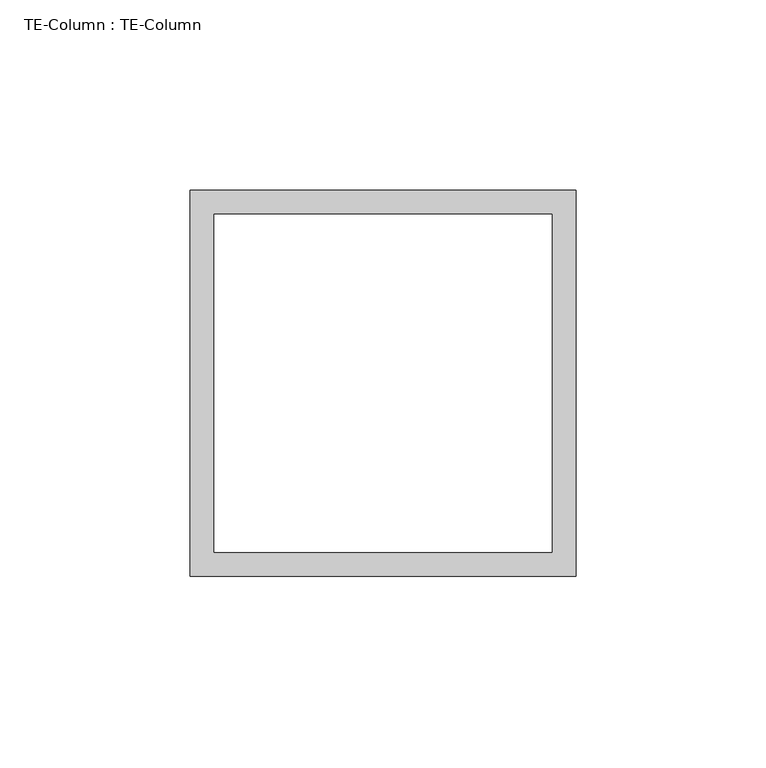
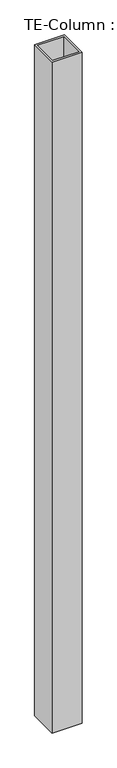
"""IFC4 building model written with IfcOpenShell, lengths in millimetres: proxy geometry, TE-Column : TE-Column."""

import ifcopenshell
import ifcopenshell.guid

model = None  # the IFC model being written
_history = None  # IfcOwnerHistory: only IFC2X3 demands one
_inside = {}  # id of a spatial element -> (the spatial element, [elements in it])
_under = {}  # id of a project, library or spatial element -> (it, [spatial elements below it])
_declared = {}  # id of a project -> (the project, [libraries it declares])
_typed = {}  # id of a type object -> (the type object, [elements of that type])
_made_of = {}  # id of a material, layer set ... -> (it, [elements and type objects made of it])


def new_model(schema):
    """Start an empty IFC model of exactly this schema.

    Asked for "IFC4X3", IfcOpenShell would pick the latest addendum, in which some entities
    have other attributes; the version numbers below select the first issue.
    IFC2X3 requires an IfcOwnerHistory on every rooted entity: one is made here for all.
    """
    global model, _history
    if schema == "IFC4X3":
        model = ifcopenshell.file(schema_version=(4, 3, 0, 0))
    else:
        model = ifcopenshell.file(schema=schema)
    _inside.clear()
    _under.clear()
    _declared.clear()
    _typed.clear()
    _made_of.clear()
    _history = None
    if model.schema == "IFC2X3":
        org = make("IfcOrganization", Name="unknown")
        user = make(
            "IfcPersonAndOrganization",
            ThePerson=make("IfcPerson", FamilyName="unknown"),
            TheOrganization=org,
        )
        app = make(
            "IfcApplication",
            ApplicationDeveloper=org,
            Version="unknown",
            ApplicationFullName="unknown",
            ApplicationIdentifier="unknown",
        )
        _history = make(
            "IfcOwnerHistory",
            OwningUser=user,
            OwningApplication=app,
            ChangeAction="ADDED",
            CreationDate=0,
        )
    return model


def make(cls, **values):
    """One entity of the class cls with the attributes given. An attribute that is None is left unset."""
    return model.create_entity(
        cls, **{name: value for name, value in values.items() if value is not None}
    )


def rooted(cls, **values):
    """An entity with a GlobalId (a new one), such as an element, a storey or a relation."""
    return make(cls, GlobalId=ifcopenshell.guid.new(), OwnerHistory=_history, **values)


def si_unit(unit_type, name, prefix=None):
    """IfcSIUnit, for example si_unit("LENGTHUNIT", "METRE", prefix="MILLI")."""
    return make("IfcSIUnit", UnitType=unit_type, Prefix=prefix, Name=name)


def assignment(units):
    """IfcUnitAssignment: the units of a project."""
    return None if units is None else make("IfcUnitAssignment", Units=units)


def point(xyz):
    """IfcCartesianPoint."""
    return None if xyz is None else make("IfcCartesianPoint", Coordinates=xyz)


def direction(xyz):
    """IfcDirection."""
    return None if xyz is None else make("IfcDirection", DirectionRatios=xyz)


def frame(location, z_axis=None, x_axis=None):
    """IfcAxis2Placement3D, a coordinate frame: its origin and axes. An axis left out is left unset."""
    return make(
        "IfcAxis2Placement3D",
        Location=point(location),
        Axis=direction(z_axis),
        RefDirection=direction(x_axis),
    )


def origin():
    """The frame at (0, 0, 0) with its axes left unset."""
    return frame((0.0, 0.0, 0.0))


def place(relative_to, where):
    """IfcLocalPlacement: puts the frame where relative to a parent placement (None: the world)."""
    return make(
        "IfcLocalPlacement", PlacementRelTo=relative_to, RelativePlacement=where
    )


def context(
    kind, dimensions, precision=None, world=None, true_north=None, identifier=None
):
    """IfcGeometricRepresentationContext, for example the 3D "Model" context."""
    return make(
        "IfcGeometricRepresentationContext",
        ContextIdentifier=identifier,
        ContextType=kind,
        CoordinateSpaceDimension=dimensions,
        Precision=precision,
        WorldCoordinateSystem=world,
        TrueNorth=true_north,
    )


def project(units=None, contexts=None):
    """IfcProject with its units and contexts."""
    return rooted(
        "IfcProject",
        Name="project",
        RepresentationContexts=contexts,
        UnitsInContext=assignment(units),
    )


def spatial(cls, under=None, at=None, **own):
    """A site, building, storey or space (cls), placed at a placement, below another one or the project."""
    s = rooted(cls, ObjectPlacement=at, **own)
    if under is not None:
        _under.setdefault(under.id(), (under, []))[1].append(s)
    return s


def polyline(points):
    """IfcPolyline through the points."""
    return make("IfcPolyline", Points=[point(p) for p in points])


def outline(outer, holes=None, kind="AREA"):
    """IfcArbitraryClosedProfileDef: a profile drawn as a closed curve; with holes, ...WithVoids."""
    if holes is None:
        return make("IfcArbitraryClosedProfileDef", ProfileType=kind, OuterCurve=outer)
    return make(
        "IfcArbitraryProfileDefWithVoids",
        ProfileType=kind,
        OuterCurve=outer,
        InnerCurves=holes,
    )


def extrude(swept, where, along, depth):
    """IfcExtrudedAreaSolid: the profile swept, set in the frame where, extruded along a direction by depth."""
    return make(
        "IfcExtrudedAreaSolid",
        SweptArea=swept,
        Position=where,
        ExtrudedDirection=direction(along),
        Depth=depth,
    )


def shape(context_of_items, identifier, shape_type, items):
    """IfcShapeRepresentation: the items that make up one representation, for example the "Body"."""
    return make(
        "IfcShapeRepresentation",
        ContextOfItems=context_of_items,
        RepresentationIdentifier=identifier,
        RepresentationType=shape_type,
        Items=items,
    )


def source(mapping_origin, context_of_items, identifier, shape_type, items):
    """IfcRepresentationMap: a shape defined once, which mapped items show again and again."""
    return make(
        "IfcRepresentationMap",
        MappingOrigin=mapping_origin,
        MappedRepresentation=shape(context_of_items, identifier, shape_type, items),
    )


def transform(
    local_origin,
    x_axis=None,
    y_axis=None,
    z_axis=None,
    scale=None,
    scale2=None,
    scale3=None,
    uniform=True,
):
    """IfcCartesianTransformationOperator3D, or its non-uniform kind. x_axis, y_axis, z_axis: its Axis1, 2, 3."""
    if uniform:
        return make(
            "IfcCartesianTransformationOperator3D",
            Axis1=direction(x_axis),
            Axis2=direction(y_axis),
            LocalOrigin=point(local_origin),
            Scale=scale,
            Axis3=direction(z_axis),
        )
    return make(
        "IfcCartesianTransformationOperator3DnonUniform",
        Axis1=direction(x_axis),
        Axis2=direction(y_axis),
        LocalOrigin=point(local_origin),
        Scale=scale,
        Axis3=direction(z_axis),
        Scale2=scale2,
        Scale3=scale3,
    )


def mapped(mapping_source, mapping_target):
    """IfcMappedItem: shows the shape of a source again, moved by a transform."""
    return make(
        "IfcMappedItem", MappingSource=mapping_source, MappingTarget=mapping_target
    )


def made_of(thing, what):
    """Note that an element or type object is made of a material, layer set ...; save() writes the relation."""
    if what is not None:
        _made_of.setdefault(what.id(), (what, []))[1].append(thing)
    return thing


def element(
    cls,
    number,
    at=None,
    inside=None,
    cuts=None,
    type_object=None,
    material=None,
    context=None,
    identifier="Body",
    shape_type=None,
    held_by="IfcProductDefinitionShape",
    body=None,
    shapes=None,
    **own,
):
    """One element of the class cls, such as IfcWall. Its Tag is "e" and its number.

    at: its placement. inside: the storey or other place that contains it. cuts: it is an
    opening in that element (IfcRelVoidsElement). A single representation is given by context,
    identifier, shape_type and body (its items); several are given by shapes. held_by: the class
    of the entity that holds the representations. save() writes the other relations.
    """
    e = rooted(cls, Tag="e%d" % number, ObjectPlacement=at, **own)
    if body is not None:
        shapes = [shape(context, identifier, shape_type, body)]
    if shapes is not None:
        e.Representation = make(held_by, Representations=shapes)
    if inside is not None:
        _inside.setdefault(inside.id(), (inside, []))[1].append(e)
    if cuts is not None:
        rooted(
            "IfcRelVoidsElement", RelatingBuildingElement=cuts, RelatedOpeningElement=e
        )
    if type_object is not None:
        _typed.setdefault(type_object.id(), (type_object, []))[1].append(e)
    return made_of(e, material)


def aggregate(whole, parts):
    """IfcRelAggregates: a whole, such as a stair, and the parts it consists of."""
    return rooted("IfcRelAggregates", RelatingObject=whole, RelatedObjects=parts)


def save(model, path):
    """Write the relations noted so far, then the file.

    IfcRelAggregates (storeys below a building ...), IfcRelContainedInSpatialStructure (elements
    in a storey), IfcRelDefinesByType, IfcRelAssociatesMaterial and IfcRelDeclares: one each for
    every whole, place, type object, material and project.
    """
    for whole, parts in _under.values():
        aggregate(whole, parts)
    for where, things in _inside.values():
        rooted(
            "IfcRelContainedInSpatialStructure",
            RelatedElements=things,
            RelatingStructure=where,
        )
    for kind, things in _typed.values():
        rooted("IfcRelDefinesByType", RelatedObjects=things, RelatingType=kind)
    for what, things in _made_of.values():
        rooted("IfcRelAssociatesMaterial", RelatedObjects=things, RelatingMaterial=what)
    for by, libraries in _declared.values():
        rooted("IfcRelDeclares", RelatingContext=by, RelatedDefinitions=libraries)
    model.write(path)


def te_column_te_column_7b45b3bc(model_context):
    return source(origin(), model_context, "Body", "SweptSolid", [
        extrude(outline(polyline([(587467.4934739, -531667.7913841), (587467.4934739, -531769.3913841), (587365.8934739, -531769.3913841), (587365.8934739, -531667.7913841), (587467.4934739, -531667.7913841)]), holes=[polyline([(587372.2434739, -531674.1413841), (587372.2434739, -531763.0413841), (587461.1434739, -531763.0413841), (587461.1434739, -531674.1413841), (587372.2434739, -531674.1413841)])]), frame((0.0, 0.0, 28.575), z_axis=(0.0, 0.0, 1.0), x_axis=(1.0, 0.0, 0.0)), (0.0, 0.0, 1.0), 2406.65),
    ])


if __name__ == "__main__":
    model = new_model("IFC4")
    model_context = context("Model", 3, world=origin())
    ifc_project = project(units=[si_unit("LENGTHUNIT", "METRE", prefix="MILLI")], contexts=[model_context])
    site = spatial("IfcSite", under=ifc_project)
    building = spatial("IfcBuilding", under=site)
    placement = place(None, origin())
    te_column_te_column_shape = te_column_te_column_7b45b3bc(model_context)
    element("IfcBuildingElementProxy", 1, Name="TE-Column : TE-Column", ObjectType="TE-Column : TE-Column", at=placement, inside=building, context=model_context, shape_type="MappedRepresentation", body=[
        mapped(te_column_te_column_shape, transform((0.0, 0.0, 0.0), x_axis=(1.0, 0.0, 0.0), y_axis=(0.0, 1.0, 0.0), z_axis=(0.0, 0.0, 1.0))),
    ])
    save(model, "model.ifc")

# Revit data of these elements
# Element 1 (IfcBuildingElementProxy, "TE-Column : TE-Column")
#   Materials on its faces: "4\"X4\" GALV. HSS TUBING"
# Materials
#   "4\"X4\" GALV. HSS TUBING": class "Generic", colour RGB 211 211 207, transparency 0, Cost = 0
